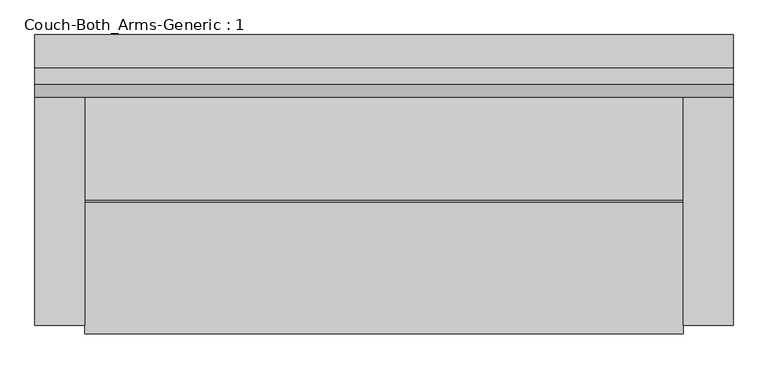
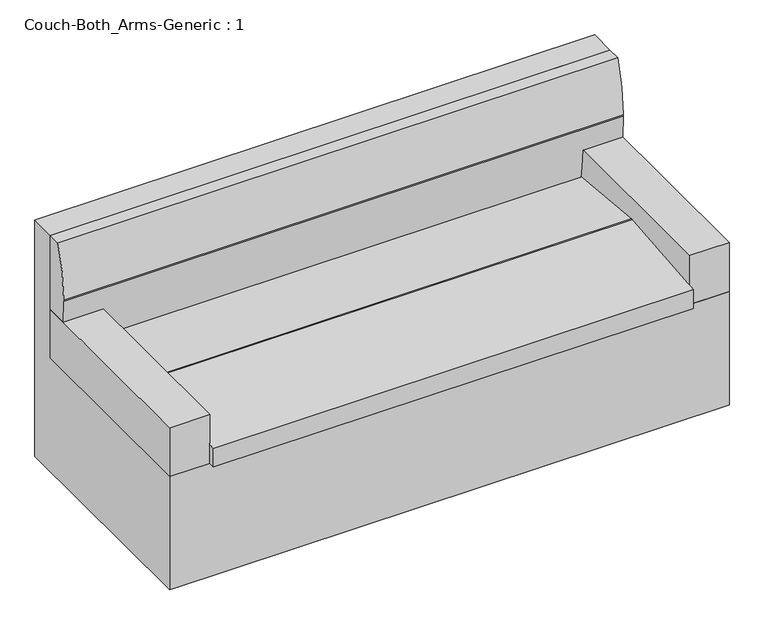
"""IFC4 building model written with IfcOpenShell, lengths in millimetres: furniture geometry, Couch-Both_Arms-Generic : 1."""

import ifcopenshell
import ifcopenshell.guid

model = None  # the IFC model being written
_history = None  # IfcOwnerHistory: only IFC2X3 demands one
_inside = {}  # id of a spatial element -> (the spatial element, [elements in it])
_under = {}  # id of a project, library or spatial element -> (it, [spatial elements below it])
_declared = {}  # id of a project -> (the project, [libraries it declares])
_typed = {}  # id of a type object -> (the type object, [elements of that type])
_made_of = {}  # id of a material, layer set ... -> (it, [elements and type objects made of it])


def new_model(schema):
    """Start an empty IFC model of exactly this schema.

    Asked for "IFC4X3", IfcOpenShell would pick the latest addendum, in which some entities
    have other attributes; the version numbers below select the first issue.
    IFC2X3 requires an IfcOwnerHistory on every rooted entity: one is made here for all.
    """
    global model, _history
    if schema == "IFC4X3":
        model = ifcopenshell.file(schema_version=(4, 3, 0, 0))
    else:
        model = ifcopenshell.file(schema=schema)
    _inside.clear()
    _under.clear()
    _declared.clear()
    _typed.clear()
    _made_of.clear()
    _history = None
    if model.schema == "IFC2X3":
        org = make("IfcOrganization", Name="unknown")
        user = make(
            "IfcPersonAndOrganization",
            ThePerson=make("IfcPerson", FamilyName="unknown"),
            TheOrganization=org,
        )
        app = make(
            "IfcApplication",
            ApplicationDeveloper=org,
            Version="unknown",
            ApplicationFullName="unknown",
            ApplicationIdentifier="unknown",
        )
        _history = make(
            "IfcOwnerHistory",
            OwningUser=user,
            OwningApplication=app,
            ChangeAction="ADDED",
            CreationDate=0,
        )
    return model


def make(cls, **values):
    """One entity of the class cls with the attributes given. An attribute that is None is left unset."""
    return model.create_entity(
        cls, **{name: value for name, value in values.items() if value is not None}
    )


def rooted(cls, **values):
    """An entity with a GlobalId (a new one), such as an element, a storey or a relation."""
    return make(cls, GlobalId=ifcopenshell.guid.new(), OwnerHistory=_history, **values)


def si_unit(unit_type, name, prefix=None):
    """IfcSIUnit, for example si_unit("LENGTHUNIT", "METRE", prefix="MILLI")."""
    return make("IfcSIUnit", UnitType=unit_type, Prefix=prefix, Name=name)


def assignment(units):
    """IfcUnitAssignment: the units of a project."""
    return None if units is None else make("IfcUnitAssignment", Units=units)


def point(xyz):
    """IfcCartesianPoint."""
    return None if xyz is None else make("IfcCartesianPoint", Coordinates=xyz)


def direction(xyz):
    """IfcDirection."""
    return None if xyz is None else make("IfcDirection", DirectionRatios=xyz)


def frame(location, z_axis=None, x_axis=None):
    """IfcAxis2Placement3D, a coordinate frame: its origin and axes. An axis left out is left unset."""
    return make(
        "IfcAxis2Placement3D",
        Location=point(location),
        Axis=direction(z_axis),
        RefDirection=direction(x_axis),
    )


def frame_2d(location, x_axis=None):
    """IfcAxis2Placement2D, a coordinate frame in the plane: its origin and x axis."""
    return make(
        "IfcAxis2Placement2D", Location=point(location), RefDirection=direction(x_axis)
    )


def origin():
    """The frame at (0, 0, 0) with its axes left unset."""
    return frame((0.0, 0.0, 0.0))


def place(relative_to, where):
    """IfcLocalPlacement: puts the frame where relative to a parent placement (None: the world)."""
    return make(
        "IfcLocalPlacement", PlacementRelTo=relative_to, RelativePlacement=where
    )


def context(
    kind, dimensions, precision=None, world=None, true_north=None, identifier=None
):
    """IfcGeometricRepresentationContext, for example the 3D "Model" context."""
    return make(
        "IfcGeometricRepresentationContext",
        ContextIdentifier=identifier,
        ContextType=kind,
        CoordinateSpaceDimension=dimensions,
        Precision=precision,
        WorldCoordinateSystem=world,
        TrueNorth=true_north,
    )


def project(units=None, contexts=None):
    """IfcProject with its units and contexts."""
    return rooted(
        "IfcProject",
        Name="project",
        RepresentationContexts=contexts,
        UnitsInContext=assignment(units),
    )


def spatial(cls, under=None, at=None, **own):
    """A site, building, storey or space (cls), placed at a placement, below another one or the project."""
    s = rooted(cls, ObjectPlacement=at, **own)
    if under is not None:
        _under.setdefault(under.id(), (under, []))[1].append(s)
    return s


def polyline(points):
    """IfcPolyline through the points."""
    return make("IfcPolyline", Points=[point(p) for p in points])


def circle_curve(where, radius):
    """IfcCircle in the frame where."""
    return make("IfcCircle", Position=where, Radius=radius)


def trimmed(basis, trim1, trim2, sense, master):
    """IfcTrimmedCurve: the piece of a basis curve between two trims."""
    return make(
        "IfcTrimmedCurve",
        BasisCurve=basis,
        Trim1=trim1,
        Trim2=trim2,
        SenseAgreement=sense,
        MasterRepresentation=master,
    )


def segment(curve, same_sense, transition):
    """IfcCompositeCurveSegment."""
    return make(
        "IfcCompositeCurveSegment",
        Transition=transition,
        SameSense=same_sense,
        ParentCurve=curve,
    )


def composite_curve(segments, self_intersect=None):
    """IfcCompositeCurve: segments joined end to end."""
    return make("IfcCompositeCurve", Segments=segments, SelfIntersect=self_intersect)


def outline(outer, holes=None, kind="AREA"):
    """IfcArbitraryClosedProfileDef: a profile drawn as a closed curve; with holes, ...WithVoids."""
    if holes is None:
        return make("IfcArbitraryClosedProfileDef", ProfileType=kind, OuterCurve=outer)
    return make(
        "IfcArbitraryProfileDefWithVoids",
        ProfileType=kind,
        OuterCurve=outer,
        InnerCurves=holes,
    )


def extrude(swept, where, along, depth):
    """IfcExtrudedAreaSolid: the profile swept, set in the frame where, extruded along a direction by depth."""
    return make(
        "IfcExtrudedAreaSolid",
        SweptArea=swept,
        Position=where,
        ExtrudedDirection=direction(along),
        Depth=depth,
    )


def shape(context_of_items, identifier, shape_type, items):
    """IfcShapeRepresentation: the items that make up one representation, for example the "Body"."""
    return make(
        "IfcShapeRepresentation",
        ContextOfItems=context_of_items,
        RepresentationIdentifier=identifier,
        RepresentationType=shape_type,
        Items=items,
    )


def source(mapping_origin, context_of_items, identifier, shape_type, items):
    """IfcRepresentationMap: a shape defined once, which mapped items show again and again."""
    return make(
        "IfcRepresentationMap",
        MappingOrigin=mapping_origin,
        MappedRepresentation=shape(context_of_items, identifier, shape_type, items),
    )


def transform(
    local_origin,
    x_axis=None,
    y_axis=None,
    z_axis=None,
    scale=None,
    scale2=None,
    scale3=None,
    uniform=True,
):
    """IfcCartesianTransformationOperator3D, or its non-uniform kind. x_axis, y_axis, z_axis: its Axis1, 2, 3."""
    if uniform:
        return make(
            "IfcCartesianTransformationOperator3D",
            Axis1=direction(x_axis),
            Axis2=direction(y_axis),
            LocalOrigin=point(local_origin),
            Scale=scale,
            Axis3=direction(z_axis),
        )
    return make(
        "IfcCartesianTransformationOperator3DnonUniform",
        Axis1=direction(x_axis),
        Axis2=direction(y_axis),
        LocalOrigin=point(local_origin),
        Scale=scale,
        Axis3=direction(z_axis),
        Scale2=scale2,
        Scale3=scale3,
    )


def mapped(mapping_source, mapping_target):
    """IfcMappedItem: shows the shape of a source again, moved by a transform."""
    return make(
        "IfcMappedItem", MappingSource=mapping_source, MappingTarget=mapping_target
    )


def made_of(thing, what):
    """Note that an element or type object is made of a material, layer set ...; save() writes the relation."""
    if what is not None:
        _made_of.setdefault(what.id(), (what, []))[1].append(thing)
    return thing


def element(
    cls,
    number,
    at=None,
    inside=None,
    cuts=None,
    type_object=None,
    material=None,
    context=None,
    identifier="Body",
    shape_type=None,
    held_by="IfcProductDefinitionShape",
    body=None,
    shapes=None,
    **own,
):
    """One element of the class cls, such as IfcWall. Its Tag is "e" and its number.

    at: its placement. inside: the storey or other place that contains it. cuts: it is an
    opening in that element (IfcRelVoidsElement). A single representation is given by context,
    identifier, shape_type and body (its items); several are given by shapes. held_by: the class
    of the entity that holds the representations. save() writes the other relations.
    """
    e = rooted(cls, Tag="e%d" % number, ObjectPlacement=at, **own)
    if body is not None:
        shapes = [shape(context, identifier, shape_type, body)]
    if shapes is not None:
        e.Representation = make(held_by, Representations=shapes)
    if inside is not None:
        _inside.setdefault(inside.id(), (inside, []))[1].append(e)
    if cuts is not None:
        rooted(
            "IfcRelVoidsElement", RelatingBuildingElement=cuts, RelatedOpeningElement=e
        )
    if type_object is not None:
        _typed.setdefault(type_object.id(), (type_object, []))[1].append(e)
    return made_of(e, material)


def aggregate(whole, parts):
    """IfcRelAggregates: a whole, such as a stair, and the parts it consists of."""
    return rooted("IfcRelAggregates", RelatingObject=whole, RelatedObjects=parts)


def save(model, path):
    """Write the relations noted so far, then the file.

    IfcRelAggregates (storeys below a building ...), IfcRelContainedInSpatialStructure (elements
    in a storey), IfcRelDefinesByType, IfcRelAssociatesMaterial and IfcRelDeclares: one each for
    every whole, place, type object, material and project.
    """
    for whole, parts in _under.values():
        aggregate(whole, parts)
    for where, things in _inside.values():
        rooted(
            "IfcRelContainedInSpatialStructure",
            RelatedElements=things,
            RelatingStructure=where,
        )
    for kind, things in _typed.values():
        rooted("IfcRelDefinesByType", RelatedObjects=things, RelatingType=kind)
    for what, things in _made_of.values():
        rooted("IfcRelAssociatesMaterial", RelatedObjects=things, RelatingMaterial=what)
    for by, libraries in _declared.values():
        rooted("IfcRelDeclares", RelatingContext=by, RelatedDefinitions=libraries)
    model.write(path)


def plane_surface(at):
    """IfcPlane: the flat surface through the origin of the frame at, square to its z axis."""
    return make("IfcPlane", Position=at)


def cylinder_surface(at, radius):
    """IfcCylindricalSurface: all points at the distance radius from the z axis of the frame at."""
    return make("IfcCylindricalSurface", Position=at, Radius=radius)


def advanced_brep(points, edges, surfaces, faces):
    """IfcAdvancedBrep: a solid bounded by faces that lie on surfaces and meet in shared edges.

    An edge is (start, end): straight between two places in points (the first is 0);
    or (start, end, curve); or (start, end, curve, False) where it runs against its curve.
    A face is (place in surfaces, loops), or (place, loops, False) where it looks against
    its surface's normal. A loop lists edges by number (the first is 1), with a minus sign
    where the edge is run from its end to its start. The first loop is the outer one.
    """
    corners = [point(p) for p in points]
    vertices = [make("IfcVertexPoint", VertexGeometry=c) for c in corners]
    made = []
    for start, end, *more in edges:
        made.append(
            make(
                "IfcEdgeCurve",
                EdgeStart=vertices[start],
                EdgeEnd=vertices[end],
                EdgeGeometry=more[0] if more else make("IfcPolyline", Points=[corners[start], corners[end]]),
                SameSense=more[1] if len(more) > 1 else True,
            )
        )
    hull = []
    for where, loops, *sense in faces:
        bounds = []
        for j, loop in enumerate(loops):
            ring = [make("IfcOrientedEdge", EdgeElement=made[abs(k) - 1], Orientation=k > 0) for k in loop]
            bounds.append(
                make(
                    "IfcFaceOuterBound" if j == 0 else "IfcFaceBound",
                    Bound=make("IfcEdgeLoop", EdgeList=ring),
                    Orientation=True,
                )
            )
        hull.append(make("IfcAdvancedFace", Bounds=bounds, FaceSurface=surfaces[where], SameSense=sense[0] if sense else True))
    return make("IfcAdvancedBrep", Outer=make("IfcClosedShell", CfsFaces=hull))


def couch_both_arms_generic_1_b71010d0(model_context):
    return source(origin(), model_context, "Body", "SolidModel", [
        extrude(outline(composite_curve([segment(polyline([(-469.9, 457.2), (-469.9, 533.4)]), True, "CONTINUOUS"), segment(trimmed(circle_curve(frame_2d((-66.675, -1581.2822917)), 2152.7822917), [point((-469.9, 533.4))], [point((-66.675, 571.5))], False, "CARTESIAN"), True, "CONTINUOUS"), segment(polyline([(-66.675, 571.5), (-60.325, 571.5)]), True, "CONTINUOUS"), segment(trimmed(circle_curve(frame_2d((-60.325, -1581.2822917)), 2152.7822917), [point((-60.325, 571.5))], [point((342.9, 533.4))], False, "CARTESIAN"), True, "CONTINUOUS"), segment(polyline([(342.9, 533.4), (342.9, 457.2), (-469.9, 457.2)]), True, "CONTINUOUS")], self_intersect=False)), frame((-914.4, 0.0, 0.0), z_axis=(1.0, 0.0, 0.0), x_axis=(0.0, 1.0, 0.0)), (0.0, 0.0, 1.0), 1828.8),
        extrude(outline(polyline([(-914.4, 342.9), (-914.4, -444.5), (-1066.8, -444.5), (-1066.8, 342.9), (-914.4, 342.9)])), frame((0.0, 0.0, 457.2), z_axis=(0.0, 0.0, 1.0), x_axis=(1.0, 0.0, 0.0)), (0.0, 0.0, 1.0), 196.85),
        extrude(outline(polyline([(1066.8, 342.9), (1066.8, -444.5), (914.4, -444.5), (914.4, 342.9), (1066.8, 342.9)])), frame((0.0, 0.0, 457.2), z_axis=(0.0, 0.0, 1.0), x_axis=(1.0, 0.0, 0.0)), (0.0, 0.0, 1.0), 196.85),
        advanced_brep(
        [(1066.8, 292.1, 952.5), (1066.8, 254.0, 746.125), (1066.8, 254.0, 739.775), (1066.8, 257.0484243, 654.05), (1066.8, 342.9, 654.05), (1066.8, 342.9, 952.5), (-1066.8, 254.0, 739.775), (-1066.8, 254.0, 746.125), (-1066.8, 292.1, 952.5), (-1066.8, 342.9, 952.5), (-1066.8, 342.9, 654.05), (-1066.8, 257.0484243, 654.05), (-914.4, 257.0484243, 654.05), (-914.4, 271.7760797, 533.4), (914.4, 271.7760797, 533.4), (914.4, 257.0484243, 654.05), (914.4, 342.9, 533.4), (-914.4, 342.9, 533.4), (914.4, 342.9, 654.05), (-914.4, 342.9, 654.05)],
        [
            (0, 1, circle_curve(frame((1066.8, 831.9822917, 746.125), z_axis=(1.0, 0.0, 0.0), x_axis=(0.0, 0.0, -1.0)), 577.9822917)),
            (1, 2),
            (2, 3, circle_curve(frame((1066.8, 1460.8642357, 739.775), z_axis=(1.0, 0.0, 0.0), x_axis=(0.0, 0.0, -1.0)), 1206.8642357)),
            (3, 4),
            (4, 5),
            (5, 0),
            (6, 7),
            (7, 8, circle_curve(frame((-1066.8, 831.9822917, 746.125), z_axis=(-1.0, 0.0, 0.0), x_axis=(0.0, 0.0, -1.0)), 577.9822917)),
            (8, 9),
            (9, 10),
            (10, 11),
            (11, 6, circle_curve(frame((-1066.8, 1460.8642357, 739.775), z_axis=(-1.0, 0.0, 0.0), x_axis=(0.0, 0.0, -1.0)), 1206.8642357)),
            (0, 8),
            (7, 1),
            (6, 2),
            (11, 12),
            (12, 13, circle_curve(frame((-914.4, 1460.8642357, 739.775), z_axis=(1.0, 0.0, 0.0), x_axis=(0.0, 0.0, -1.0)), 1206.8642357)),
            (13, 14),
            (14, 15, circle_curve(frame((914.4, 1460.8642357, 739.775), z_axis=(-1.0, 0.0, 0.0), x_axis=(0.0, 0.0, -1.0)), 1206.8642357)),
            (15, 3),
            (16, 14),
            (13, 17),
            (17, 16),
            (9, 5),
            (4, 18),
            (18, 16),
            (17, 19),
            (19, 10),
            (15, 18),
            (19, 12),
        ],
        [
            plane_surface(frame((1066.8, 271.7760797, 742.95), z_axis=(1.0, 0.0, 0.0), x_axis=(0.0, -1.0, 0.0))),
            plane_surface(frame((-1066.8, 271.7760797, 742.95), z_axis=(-1.0, 0.0, 0.0), x_axis=(0.0, -1.0, 0.0))),
            cylinder_surface(frame((1066.8, 831.9822917, 746.125), z_axis=(1.0, 0.0, 0.0), x_axis=(0.0, 0.0, -1.0)), 577.9822917),
            plane_surface(frame((1066.8, 254.0, 746.125), z_axis=(0.0, -1.0, 0.0), x_axis=(-1.0, 0.0, 0.0))),
            cylinder_surface(frame((1066.8, 1460.8642357, 739.775), z_axis=(1.0, 0.0, 0.0), x_axis=(0.0, 0.0, -1.0)), 1206.8642357),
            plane_surface(frame((1066.8, 271.7760797, 533.4), z_axis=(0.0, 0.0, -1.0), x_axis=(-1.0, 0.0, 0.0))),
            plane_surface(frame((-1066.8, 342.9, 952.5), z_axis=(0.0, 1.0, 0.0), x_axis=(1.0, 0.0, 0.0))),
            plane_surface(frame((1066.8, 292.1, 952.5), z_axis=(0.0, 0.0, 1.0), x_axis=(0.0, 1.0, 0.0))),
            plane_surface(frame((914.4, 501.65, 654.05), z_axis=(0.0, 0.0, -1.0), x_axis=(-1.0, 0.0, 0.0))),
            plane_surface(frame((914.4, 501.65, 654.05), z_axis=(1.0, 0.0, 0.0), x_axis=(0.0, 0.0, -1.0))),
            plane_surface(frame((-1066.8, 450.85, 654.05), z_axis=(0.0, 0.0, -1.0), x_axis=(-1.0, 0.0, 0.0))),
            plane_surface(frame((-914.4, 101.6, 654.05), z_axis=(-1.0, 0.0, 0.0), x_axis=(0.0, 0.0, -1.0))),
        ],
        [
            (0, [[1, 2, 3, 4, 5, 6]]),
            (1, [[7, 8, 9, 10, 11, 12]]),
            (2, [[-1, 13, -8, 14]]),
            (3, [[-2, -14, -7, 15]]),
            (4, [[-15, -12, 16, 17, 18, 19, 20, -3]]),
            (5, [[21, -18, 22, 23]]),
            (6, [[24, -5, 25, 26, -23, 27, 28, -10]]),
            (7, [[-24, -9, -13, -6]]),
            (8, [[29, -25, -4, -20]]),
            (9, [[-29, -19, -21, -26]]),
            (10, [[30, -16, -11, -28]]),
            (11, [[-30, -27, -22, -17]]),
        ],
    ),
        extrude(outline(polyline([(-444.5, 457.2), (342.9, 457.2), (342.9, 952.5), (444.5, 952.5), (444.5, 0.0), (-444.5, 0.0), (-444.5, 457.2)])), frame((-1066.8, 0.0, 0.0), z_axis=(1.0, 0.0, 0.0), x_axis=(0.0, 1.0, 0.0)), (0.0, 0.0, 1.0), 2133.6),
    ])


if __name__ == "__main__":
    model = new_model("IFC4")
    model_context = context("Model", 3, world=origin())
    ifc_project = project(units=[si_unit("LENGTHUNIT", "METRE", prefix="MILLI")], contexts=[model_context])
    site = spatial("IfcSite", under=ifc_project)
    building = spatial("IfcBuilding", under=site)
    placement = place(None, origin())
    couch_both_arms_generic_1_shape = couch_both_arms_generic_1_b71010d0(model_context)
    element("IfcFurniture", 1, ObjectType="Couch-Both_Arms-Generic : 1", at=placement, inside=building, context=model_context, shape_type="MappedRepresentation", body=[
        mapped(couch_both_arms_generic_1_shape, transform((0.0, 0.0, 0.0), x_axis=(1.0, 0.0, 0.0), y_axis=(0.0, 1.0, 0.0), z_axis=(0.0, 0.0, 1.0))),
    ])
    save(model, "model.ifc")

# Revit data of these elements
# Type "Couch-Both_Arms-Generic : 1"
#   OmniClass Title = "Settees, Sofas"
#   OmniClass Number = "23.40.20.14.14.14"
#   Model = "Both Arms"
#   Manufacturer = "Generic"
#   Description = "Straight Couch with armrests on both sides"
#   Width = 7' - 0"
#   Seat Height = 1' - 6"
#   Height = 3' - 1 1/2"
#   Depth = 2' - 11"
#   Couch Cushion Width = 6' - 0"
#   Couch Cushion Depth = 2' - 8"
#   Backseat Height = 1' - 4 1/2"
#   Arm Rest Width = 0' - 6"
#   Arm Rest Depth = 2' - 7"
#   Surface Finish = none
#   Type Comments = ""
#   Keynote = ""
#   Assembly Code = ""
# Element 1 (IfcFurniture, "Couch-Both_Arms-Generic : 1")
#   Materials on its faces: "MAX HEIGHT OF  COUNTERTOP 34\""
# Materials
#   "MAX HEIGHT OF  COUNTERTOP 34\"": class "Generic", colour RGB 181 181 181, transparency 0, Cost = 0
